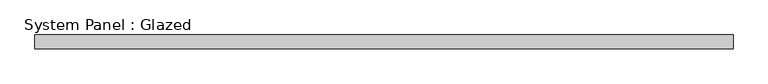
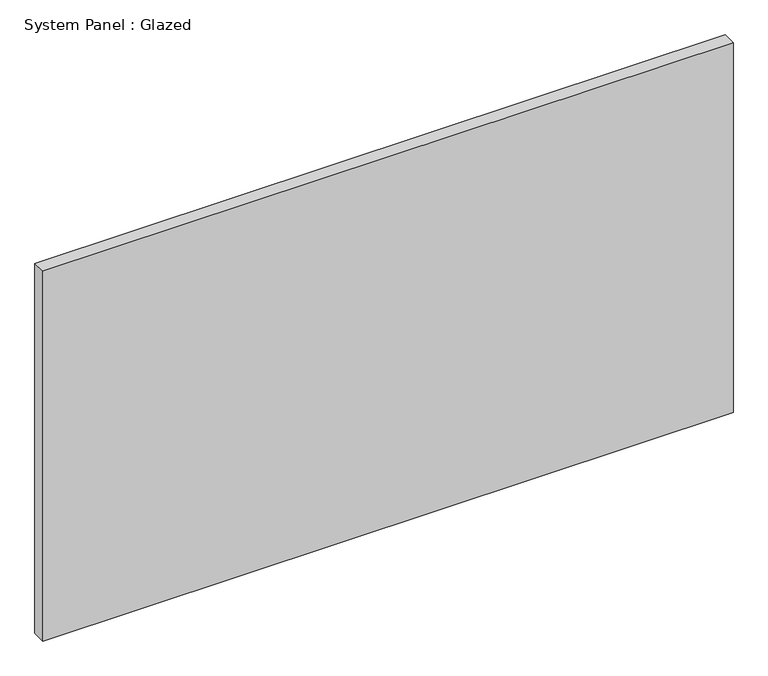
"""IFC4 building model written with IfcOpenShell, lengths in millimetres: plate geometry, System Panel : Glazed."""

from ifc_helpers import new_model, si_unit, origin, origin_with_axes, place, context, project, spatial, polyline, outline, extrude, source, transform, mapped, element, save


def system_panel_glazed_74448b90(model_context):
    return source(origin(), model_context, "Body", "SweptSolid", [
        extrude(outline(polyline([(639.2857142, 24.5), (-639.2857142, 24.5), (-639.2857142, 49.5), (639.2857142, 49.5), (639.2857142, 24.5)])), origin_with_axes(), (0.0, 0.0, 1.0), 725.0),
    ])


if __name__ == "__main__":
    model = new_model("IFC4")
    model_context = context("Model", 3, world=origin())
    ifc_project = project(units=[si_unit("LENGTHUNIT", "METRE", prefix="MILLI")], contexts=[model_context])
    site = spatial("IfcSite", under=ifc_project)
    building = spatial("IfcBuilding", under=site)
    placement = place(None, origin())
    system_panel_glazed_shape = system_panel_glazed_74448b90(model_context)
    element("IfcPlate", 1, ObjectType="System Panel : Glazed", at=placement, inside=building, context=model_context, shape_type="MappedRepresentation", body=[
        mapped(system_panel_glazed_shape, transform((0.0, 0.0, 0.0), x_axis=(1.0, 0.0, 0.0), y_axis=(0.0, 1.0, 0.0), z_axis=(0.0, 0.0, 1.0))),
    ])
    save(model, "model.ifc")

# Revit data of these elements
# Type "System Panel : Glazed"
#   Construction Type Id = "GSP4R"
#   Analytic Construction = "1/8 in Pilkington single glazing"
#   Visual Light Transmittance = 0.9
#   Solar Heat Gain Coefficient = 0.86
#   Heat Transfer Coefficient (U) = 6.7069 W/(m²·K)
#   Define Thermal Properties by = 1
# Element 1 (IfcPlate, "System Panel : Glazed")
#   Materials on its faces: "Glass"
# Materials
#   "Glass": class "Glass", colour RGB 0 128 192, transparency 0.75, Description = "Soda Lime Glass", Cost = 0
